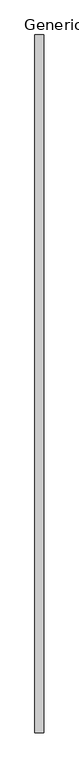
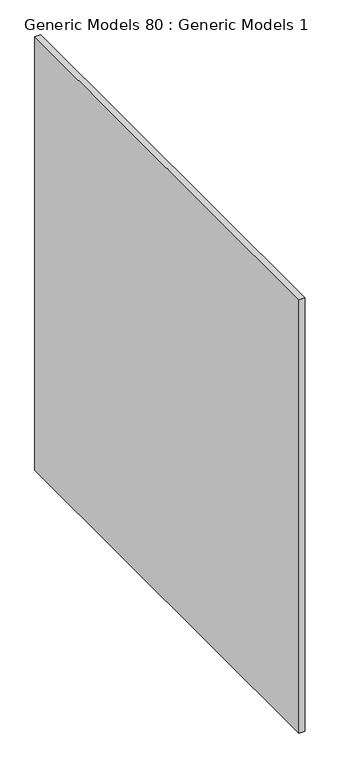
"""IFC4 building model written with IfcOpenShell, lengths in millimetres: proxy geometry, Generic Models 80 : Generic Models 1."""

import ifcopenshell
import ifcopenshell.guid

model = None  # the IFC model being written
_history = None  # IfcOwnerHistory: only IFC2X3 demands one
_inside = {}  # id of a spatial element -> (the spatial element, [elements in it])
_under = {}  # id of a project, library or spatial element -> (it, [spatial elements below it])
_declared = {}  # id of a project -> (the project, [libraries it declares])
_typed = {}  # id of a type object -> (the type object, [elements of that type])
_made_of = {}  # id of a material, layer set ... -> (it, [elements and type objects made of it])


def new_model(schema):
    """Start an empty IFC model of exactly this schema.

    Asked for "IFC4X3", IfcOpenShell would pick the latest addendum, in which some entities
    have other attributes; the version numbers below select the first issue.
    IFC2X3 requires an IfcOwnerHistory on every rooted entity: one is made here for all.
    """
    global model, _history
    if schema == "IFC4X3":
        model = ifcopenshell.file(schema_version=(4, 3, 0, 0))
    else:
        model = ifcopenshell.file(schema=schema)
    _inside.clear()
    _under.clear()
    _declared.clear()
    _typed.clear()
    _made_of.clear()
    _history = None
    if model.schema == "IFC2X3":
        org = make("IfcOrganization", Name="unknown")
        user = make(
            "IfcPersonAndOrganization",
            ThePerson=make("IfcPerson", FamilyName="unknown"),
            TheOrganization=org,
        )
        app = make(
            "IfcApplication",
            ApplicationDeveloper=org,
            Version="unknown",
            ApplicationFullName="unknown",
            ApplicationIdentifier="unknown",
        )
        _history = make(
            "IfcOwnerHistory",
            OwningUser=user,
            OwningApplication=app,
            ChangeAction="ADDED",
            CreationDate=0,
        )
    return model


def make(cls, **values):
    """One entity of the class cls with the attributes given. An attribute that is None is left unset."""
    return model.create_entity(
        cls, **{name: value for name, value in values.items() if value is not None}
    )


def rooted(cls, **values):
    """An entity with a GlobalId (a new one), such as an element, a storey or a relation."""
    return make(cls, GlobalId=ifcopenshell.guid.new(), OwnerHistory=_history, **values)


def si_unit(unit_type, name, prefix=None):
    """IfcSIUnit, for example si_unit("LENGTHUNIT", "METRE", prefix="MILLI")."""
    return make("IfcSIUnit", UnitType=unit_type, Prefix=prefix, Name=name)


def assignment(units):
    """IfcUnitAssignment: the units of a project."""
    return None if units is None else make("IfcUnitAssignment", Units=units)


def point(xyz):
    """IfcCartesianPoint."""
    return None if xyz is None else make("IfcCartesianPoint", Coordinates=xyz)


def direction(xyz):
    """IfcDirection."""
    return None if xyz is None else make("IfcDirection", DirectionRatios=xyz)


def frame(location, z_axis=None, x_axis=None):
    """IfcAxis2Placement3D, a coordinate frame: its origin and axes. An axis left out is left unset."""
    return make(
        "IfcAxis2Placement3D",
        Location=point(location),
        Axis=direction(z_axis),
        RefDirection=direction(x_axis),
    )


def origin():
    """The frame at (0, 0, 0) with its axes left unset."""
    return frame((0.0, 0.0, 0.0))


def place(relative_to, where):
    """IfcLocalPlacement: puts the frame where relative to a parent placement (None: the world)."""
    return make(
        "IfcLocalPlacement", PlacementRelTo=relative_to, RelativePlacement=where
    )


def context(
    kind, dimensions, precision=None, world=None, true_north=None, identifier=None
):
    """IfcGeometricRepresentationContext, for example the 3D "Model" context."""
    return make(
        "IfcGeometricRepresentationContext",
        ContextIdentifier=identifier,
        ContextType=kind,
        CoordinateSpaceDimension=dimensions,
        Precision=precision,
        WorldCoordinateSystem=world,
        TrueNorth=true_north,
    )


def project(units=None, contexts=None):
    """IfcProject with its units and contexts."""
    return rooted(
        "IfcProject",
        Name="project",
        RepresentationContexts=contexts,
        UnitsInContext=assignment(units),
    )


def spatial(cls, under=None, at=None, **own):
    """A site, building, storey or space (cls), placed at a placement, below another one or the project."""
    s = rooted(cls, ObjectPlacement=at, **own)
    if under is not None:
        _under.setdefault(under.id(), (under, []))[1].append(s)
    return s


def polyline(points):
    """IfcPolyline through the points."""
    return make("IfcPolyline", Points=[point(p) for p in points])


def outline(outer, holes=None, kind="AREA"):
    """IfcArbitraryClosedProfileDef: a profile drawn as a closed curve; with holes, ...WithVoids."""
    if holes is None:
        return make("IfcArbitraryClosedProfileDef", ProfileType=kind, OuterCurve=outer)
    return make(
        "IfcArbitraryProfileDefWithVoids",
        ProfileType=kind,
        OuterCurve=outer,
        InnerCurves=holes,
    )


def extrude(swept, where, along, depth):
    """IfcExtrudedAreaSolid: the profile swept, set in the frame where, extruded along a direction by depth."""
    return make(
        "IfcExtrudedAreaSolid",
        SweptArea=swept,
        Position=where,
        ExtrudedDirection=direction(along),
        Depth=depth,
    )


def shape(context_of_items, identifier, shape_type, items):
    """IfcShapeRepresentation: the items that make up one representation, for example the "Body"."""
    return make(
        "IfcShapeRepresentation",
        ContextOfItems=context_of_items,
        RepresentationIdentifier=identifier,
        RepresentationType=shape_type,
        Items=items,
    )


def source(mapping_origin, context_of_items, identifier, shape_type, items):
    """IfcRepresentationMap: a shape defined once, which mapped items show again and again."""
    return make(
        "IfcRepresentationMap",
        MappingOrigin=mapping_origin,
        MappedRepresentation=shape(context_of_items, identifier, shape_type, items),
    )


def transform(
    local_origin,
    x_axis=None,
    y_axis=None,
    z_axis=None,
    scale=None,
    scale2=None,
    scale3=None,
    uniform=True,
):
    """IfcCartesianTransformationOperator3D, or its non-uniform kind. x_axis, y_axis, z_axis: its Axis1, 2, 3."""
    if uniform:
        return make(
            "IfcCartesianTransformationOperator3D",
            Axis1=direction(x_axis),
            Axis2=direction(y_axis),
            LocalOrigin=point(local_origin),
            Scale=scale,
            Axis3=direction(z_axis),
        )
    return make(
        "IfcCartesianTransformationOperator3DnonUniform",
        Axis1=direction(x_axis),
        Axis2=direction(y_axis),
        LocalOrigin=point(local_origin),
        Scale=scale,
        Axis3=direction(z_axis),
        Scale2=scale2,
        Scale3=scale3,
    )


def mapped(mapping_source, mapping_target):
    """IfcMappedItem: shows the shape of a source again, moved by a transform."""
    return make(
        "IfcMappedItem", MappingSource=mapping_source, MappingTarget=mapping_target
    )


def made_of(thing, what):
    """Note that an element or type object is made of a material, layer set ...; save() writes the relation."""
    if what is not None:
        _made_of.setdefault(what.id(), (what, []))[1].append(thing)
    return thing


def element(
    cls,
    number,
    at=None,
    inside=None,
    cuts=None,
    type_object=None,
    material=None,
    context=None,
    identifier="Body",
    shape_type=None,
    held_by="IfcProductDefinitionShape",
    body=None,
    shapes=None,
    **own,
):
    """One element of the class cls, such as IfcWall. Its Tag is "e" and its number.

    at: its placement. inside: the storey or other place that contains it. cuts: it is an
    opening in that element (IfcRelVoidsElement). A single representation is given by context,
    identifier, shape_type and body (its items); several are given by shapes. held_by: the class
    of the entity that holds the representations. save() writes the other relations.
    """
    e = rooted(cls, Tag="e%d" % number, ObjectPlacement=at, **own)
    if body is not None:
        shapes = [shape(context, identifier, shape_type, body)]
    if shapes is not None:
        e.Representation = make(held_by, Representations=shapes)
    if inside is not None:
        _inside.setdefault(inside.id(), (inside, []))[1].append(e)
    if cuts is not None:
        rooted(
            "IfcRelVoidsElement", RelatingBuildingElement=cuts, RelatedOpeningElement=e
        )
    if type_object is not None:
        _typed.setdefault(type_object.id(), (type_object, []))[1].append(e)
    return made_of(e, material)


def aggregate(whole, parts):
    """IfcRelAggregates: a whole, such as a stair, and the parts it consists of."""
    return rooted("IfcRelAggregates", RelatingObject=whole, RelatedObjects=parts)


def save(model, path):
    """Write the relations noted so far, then the file.

    IfcRelAggregates (storeys below a building ...), IfcRelContainedInSpatialStructure (elements
    in a storey), IfcRelDefinesByType, IfcRelAssociatesMaterial and IfcRelDeclares: one each for
    every whole, place, type object, material and project.
    """
    for whole, parts in _under.values():
        aggregate(whole, parts)
    for where, things in _inside.values():
        rooted(
            "IfcRelContainedInSpatialStructure",
            RelatedElements=things,
            RelatingStructure=where,
        )
    for kind, things in _typed.values():
        rooted("IfcRelDefinesByType", RelatedObjects=things, RelatingType=kind)
    for what, things in _made_of.values():
        rooted("IfcRelAssociatesMaterial", RelatedObjects=things, RelatingMaterial=what)
    for by, libraries in _declared.values():
        rooted("IfcRelDeclares", RelatingContext=by, RelatedDefinitions=libraries)
    model.write(path)


def generic_models_80_generic_models_1_dd39fccb(model_context):
    return source(origin(), model_context, "Body", "SweptSolid", [
        extrude(outline(polyline([(46951.7485531, 1219.2), (46951.7485531, 0.0), (46935.8735531, 0.0), (46935.8735531, 1219.2), (46951.7485531, 1219.2)])), frame((0.0, 0.0, -219.626067), z_axis=(0.0, 0.0, 1.0), x_axis=(1.0, 0.0, 0.0)), (0.0, 0.0, 1.0), 1219.2),
    ])


if __name__ == "__main__":
    model = new_model("IFC4")
    model_context = context("Model", 3, world=origin())
    ifc_project = project(units=[si_unit("LENGTHUNIT", "METRE", prefix="MILLI")], contexts=[model_context])
    site = spatial("IfcSite", under=ifc_project)
    building = spatial("IfcBuilding", under=site)
    placement = place(None, origin())
    generic_models_80_generic_models_1_shape = generic_models_80_generic_models_1_dd39fccb(model_context)
    element("IfcBuildingElementProxy", 1, Name="Generic Models 80 : Generic Models 1", ObjectType="Generic Models 80 : Generic Models 1", at=placement, inside=building, context=model_context, shape_type="MappedRepresentation", body=[
        mapped(generic_models_80_generic_models_1_shape, transform((0.0, 0.0, 0.0), x_axis=(1.0, 0.0, 0.0), y_axis=(0.0, 1.0, 0.0), z_axis=(0.0, 0.0, 1.0))),
    ])
    save(model, "model.ifc")

# Revit data of these elements
# Element 1 (IfcBuildingElementProxy, "Generic Models 80 : Generic Models 1")
#   Materials on its faces: "5/8\" GYP. BD"
# Materials
#   "5/8\" GYP. BD": class "Generic", colour RGB 255 255 255, transparency 0, Description = "Gypsum Wall Board", Cost = 0
